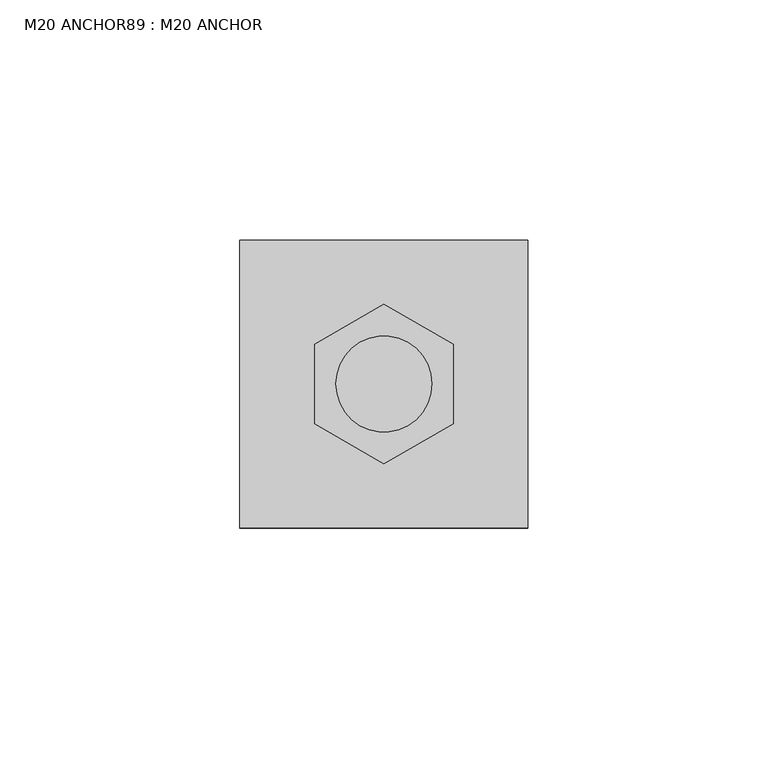
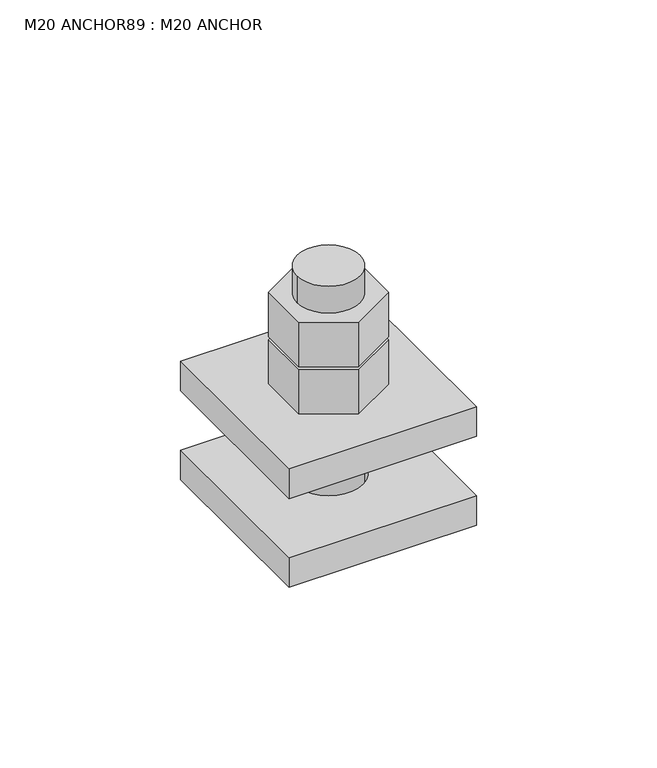
"""IFC4 building model written with IfcOpenShell, lengths in millimetres: fastener geometry, M20 ANCHOR89 : M20 ANCHOR."""

from ifc_helpers import new_model, si_unit, point, frame, frame_2d, origin, place, context, project, spatial, polyline, circle_curve, trimmed, segment, composite_curve, outline, extrude, source, transform, mapped, element, save


def m20_anchor89_m20_anchor_0efb614e(model_context):
    return source(origin(), model_context, "Body", "SweptSolid", [
        extrude(outline(polyline([(15008.0855968, 25545.0952779), (15022.4937158, 25553.4138093), (15036.9018348, 25545.0952779), (15036.9018348, 25528.4582151), (15022.4937158, 25520.1396837), (15008.0855968, 25528.4582151), (15008.0855968, 25545.0952779)]), holes=[composite_curve([segment(trimmed(circle_curve(frame_2d((15022.4937158, 25536.7767465)), 10.0), [point((15032.4937158, 25536.7767465))], [point((15012.4937158, 25536.7767465))], True, "CARTESIAN"), True, "CONTINUOUS"), segment(trimmed(circle_curve(frame_2d((15022.4937158, 25536.7767465)), 10.0), [point((15012.4937158, 25536.7767465))], [point((15032.4937158, 25536.7767465))], True, "CARTESIAN"), True, "CONTINUOUS")], self_intersect=False)]), frame((0.0, 0.0, 246.0), z_axis=(0.0, 0.0, 1.0), x_axis=(1.0, 0.0, 0.0)), (0.0, 0.0, 1.0), 15.0),
        extrude(outline(polyline([(15008.0855968, 25545.0952779), (15022.4937158, 25553.4138093), (15036.9018348, 25545.0952779), (15036.9018348, 25528.4582151), (15022.4937158, 25520.1396837), (15008.0855968, 25528.4582151), (15008.0855968, 25545.0952779)]), holes=[composite_curve([segment(trimmed(circle_curve(frame_2d((15022.4937158, 25536.7767465)), 10.0), [point((15032.4937158, 25536.7767465))], [point((15012.4937158, 25536.7767465))], True, "CARTESIAN"), True, "CONTINUOUS"), segment(trimmed(circle_curve(frame_2d((15022.4937158, 25536.7767465)), 10.0), [point((15012.4937158, 25536.7767465))], [point((15032.4937158, 25536.7767465))], True, "CARTESIAN"), True, "CONTINUOUS")], self_intersect=False)]), frame((0.0, 0.0, 230.0), z_axis=(0.0, 0.0, 1.0), x_axis=(1.0, 0.0, 0.0)), (0.0, 0.0, 1.0), 15.0),
        extrude(outline(composite_curve([segment(trimmed(circle_curve(frame_2d((15022.4937158, 25536.7767465)), 10.0), [point((15032.4937158, 25536.7767465))], [point((15012.4937158, 25536.7767465))], False, "CARTESIAN"), True, "CONTINUOUS"), segment(trimmed(circle_curve(frame_2d((15022.4937158, 25536.7767465)), 10.0), [point((15012.4937158, 25536.7767465))], [point((15032.4937158, 25536.7767465))], False, "CARTESIAN"), True, "CONTINUOUS")], self_intersect=False)), frame((0.0, 0.0, 190.0), z_axis=(0.0, 0.0, 1.0), x_axis=(1.0, 0.0, 0.0)), (0.0, 0.0, 1.0), 80.0),
        extrude(outline(polyline([(14992.4937158, 25566.7767465), (15052.4937158, 25566.7767465), (15052.4937158, 25506.7767465), (14992.4937158, 25506.7767465), (14992.4937158, 25566.7767465)]), holes=[composite_curve([segment(trimmed(circle_curve(frame_2d((15022.4937158, 25536.7767465)), 11.0), [point((15033.4937158, 25536.7767465))], [point((15011.4937158, 25536.7767465))], True, "CARTESIAN"), True, "CONTINUOUS"), segment(trimmed(circle_curve(frame_2d((15022.4937158, 25536.7767465)), 11.0), [point((15011.4937158, 25536.7767465))], [point((15033.4937158, 25536.7767465))], True, "CARTESIAN"), True, "CONTINUOUS")], self_intersect=False)]), frame((0.0, 0.0, 190.0), z_axis=(0.0, 0.0, 1.0), x_axis=(1.0, 0.0, 0.0)), (0.0, 0.0, 1.0), 10.0),
        extrude(outline(polyline([(14992.4937158, 25566.7767465), (15052.4937158, 25566.7767465), (15052.4937158, 25506.7767465), (14992.4937158, 25506.7767465), (14992.4937158, 25566.7767465)]), holes=[composite_curve([segment(trimmed(circle_curve(frame_2d((15022.4937158, 25536.7767465)), 11.0), [point((15033.4937158, 25536.7767465))], [point((15011.4937158, 25536.7767465))], True, "CARTESIAN"), True, "CONTINUOUS"), segment(trimmed(circle_curve(frame_2d((15022.4937158, 25536.7767465)), 11.0), [point((15011.4937158, 25536.7767465))], [point((15033.4937158, 25536.7767465))], True, "CARTESIAN"), True, "CONTINUOUS")], self_intersect=False)]), frame((0.0, 0.0, 220.0), z_axis=(0.0, 0.0, 1.0), x_axis=(1.0, 0.0, 0.0)), (0.0, 0.0, 1.0), 10.0),
    ])


if __name__ == "__main__":
    model = new_model("IFC4")
    model_context = context("Model", 3, world=origin())
    ifc_project = project(units=[si_unit("LENGTHUNIT", "METRE", prefix="MILLI")], contexts=[model_context])
    site = spatial("IfcSite", under=ifc_project)
    building = spatial("IfcBuilding", under=site)
    placement = place(None, origin())
    m20_anchor89_m20_anchor_shape = m20_anchor89_m20_anchor_0efb614e(model_context)
    element("IfcFastener", 1, ObjectType="M20 ANCHOR89 : M20 ANCHOR", at=placement, inside=building, context=model_context, shape_type="MappedRepresentation", body=[
        mapped(m20_anchor89_m20_anchor_shape, transform((0.0, 0.0, 0.0), x_axis=(1.0, 0.0, 0.0), y_axis=(0.0, 1.0, 0.0), z_axis=(0.0, 0.0, 1.0))),
    ])
    save(model, "model.ifc")
